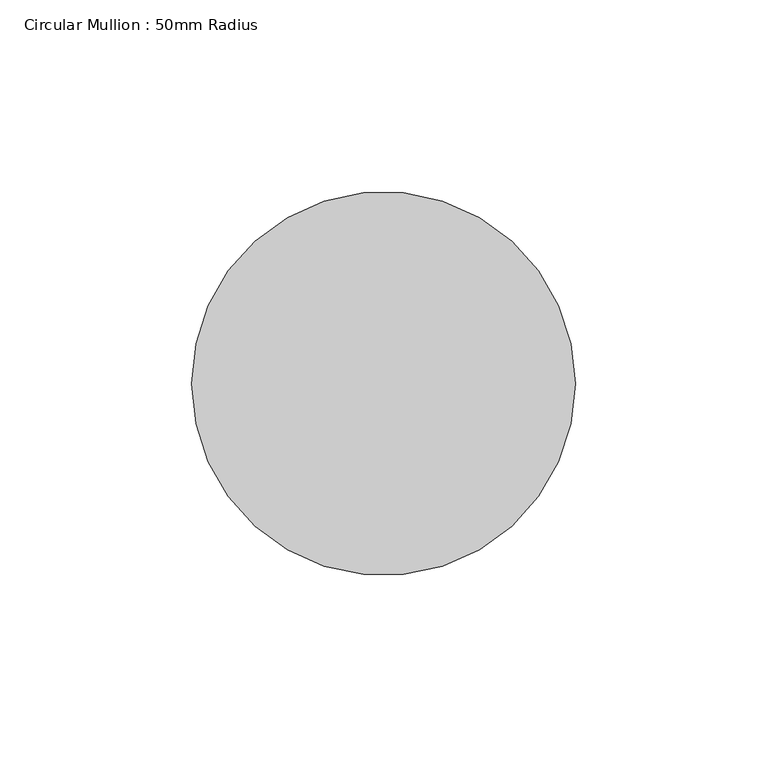
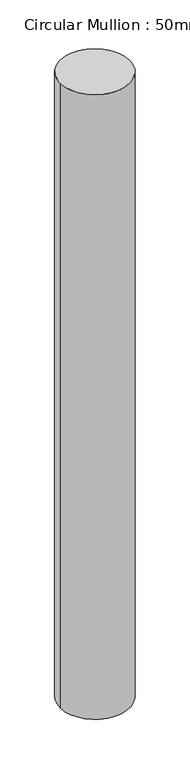
"""IFC4 building model written with IfcOpenShell, lengths in millimetres: member geometry, Circular Mullion : 50mm Radius."""

from ifc_helpers import new_model, si_unit, point, frame, origin, origin_2d, place, context, project, spatial, circle_curve, trimmed, segment, composite_curve, outline, extrude, source, transform, mapped, element, save


def circular_mullion_50mm_radius_5296bf16(model_context):
    return source(origin(), model_context, "Body", "SweptSolid", [
        extrude(outline(composite_curve([segment(trimmed(circle_curve(origin_2d(), 50.0), [point((50.0, 0.0))], [point((-50.0, 0.0))], False, "CARTESIAN"), True, "CONTINUOUS"), segment(trimmed(circle_curve(origin_2d(), 50.0), [point((-50.0, 0.0))], [point((50.0, 0.0))], False, "CARTESIAN"), True, "CONTINUOUS")], self_intersect=False)), frame((0.0, 0.0, -948.6961445), z_axis=(0.0, 0.0, 1.0), x_axis=(1.0, 0.0, 0.0)), (0.0, 0.0, 1.0), 948.6961445),
    ])


if __name__ == "__main__":
    model = new_model("IFC4")
    model_context = context("Model", 3, world=origin())
    ifc_project = project(units=[si_unit("LENGTHUNIT", "METRE", prefix="MILLI")], contexts=[model_context])
    site = spatial("IfcSite", under=ifc_project)
    building = spatial("IfcBuilding", under=site)
    placement = place(None, origin())
    circular_mullion_50mm_radius_shape = circular_mullion_50mm_radius_5296bf16(model_context)
    element("IfcMember", 1, ObjectType="Circular Mullion : 50mm Radius", at=placement, inside=building, context=model_context, shape_type="MappedRepresentation", body=[
        mapped(circular_mullion_50mm_radius_shape, transform((0.0, 0.0, 0.0), x_axis=(1.0, 0.0, 0.0), y_axis=(0.0, 1.0, 0.0), z_axis=(0.0, 0.0, 1.0))),
    ])
    save(model, "model.ifc")

# Revit data of these elements
# Type "Circular Mullion : 50mm Radius"
#   built-in parameter 1007350 = 0.164042 (stored number, unit not read)
# Element 1 (IfcMember, "Circular Mullion : 50mm Radius")
#   Materials on its faces: "Aluminium"
# Materials
#   "Aluminium": class "Metal", colour RGB 247 247 247, transparency 0, Description = "Aluminium 6061", Cost = 0
